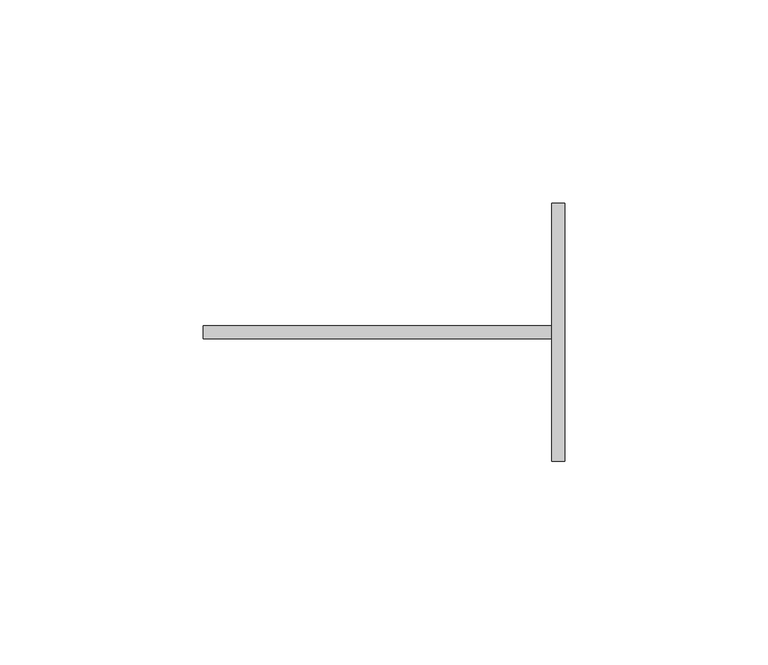
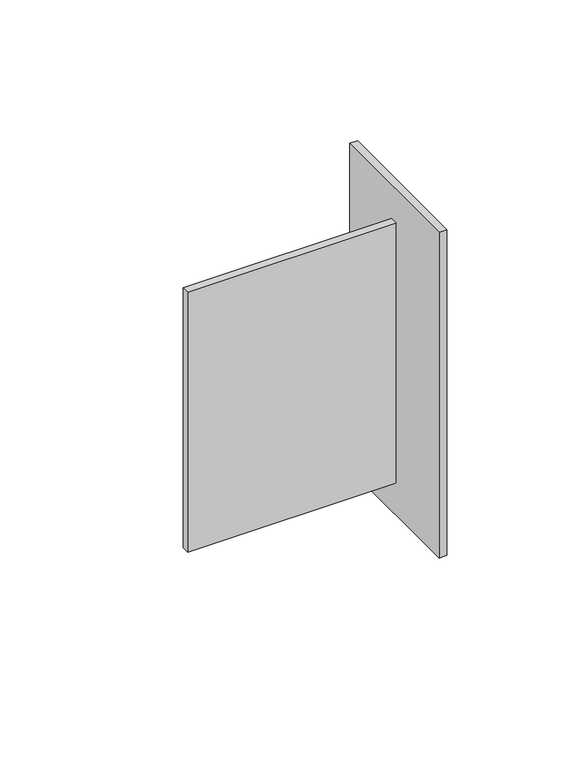
"""IFC4 building model written with IfcOpenShell, lengths in millimetres: proxy geometry, 060523 - W_P_C - Fastenings - Concealed Joist Ties:060523 - W_P_C - Fastenings - Concealed Joist Ties:154100 : 060523 - W_P_C - Fastenings - Concealed Joist Ties:060523 - W_P_C - Fastenings - Concealed Joist Ties:154100."""

from ifc_helpers import new_model, si_unit, frame, origin, place, context, project, spatial, polyline, outline, extrude, source, transform, mapped, element, save


def generic_models_267029ac(model_context):
    return source(origin(), model_context, "Body", "SweptSolid", [
        extrude(outline(polyline([(-6667.621787, -3916.4007855), (-6667.621787, -3852.9007855), (-6664.446787, -3852.9007855), (-6664.446787, -3916.4007855), (-6667.621787, -3916.4007855)])), frame((0.0, 0.0, 3169.0018876), z_axis=(0.0, 0.0, 1.0), x_axis=(1.0, 0.0, 0.0)), (0.0, 0.0, 1.0), 141.2875),
        extrude(outline(polyline([(-6753.346787, -3886.2382855), (-6753.346787, -3883.0632855), (-6667.621787, -3883.0632855), (-6667.621787, -3886.2382855), (-6753.346787, -3886.2382855)])), frame((0.0, 0.0, 3183.2893876), z_axis=(0.0, 0.0, 1.0), x_axis=(1.0, 0.0, 0.0)), (0.0, 0.0, 1.0), 112.7125),
    ])


if __name__ == "__main__":
    model = new_model("IFC4")
    model_context = context("Model", 3, world=origin())
    ifc_project = project(units=[si_unit("LENGTHUNIT", "METRE", prefix="MILLI")], contexts=[model_context])
    site = spatial("IfcSite", under=ifc_project)
    building = spatial("IfcBuilding", under=site)
    placement = place(None, origin())
    generic_models_shape = generic_models_267029ac(model_context)
    element("IfcBuildingElementProxy", 1, Name="060523 - W_P_C - Fastenings - Concealed Joist Ties:060523 - W_P_C - Fastenings - Concealed Joist Ties:154100 : 060523 - W_P_C - Fastenings - Concealed Joist Ties:060523 - W_P_C - Fastenings - Concealed Joist Ties:154100", ObjectType="060523 - W_P_C - Fastenings - Concealed Joist Ties:060523 - W_P_C - Fastenings - Concealed Joist Ties:154100 : 060523 - W_P_C - Fastenings - Concealed Joist Ties:060523 - W_P_C - Fastenings - Concealed Joist Ties:154100", at=placement, inside=building, context=model_context, shape_type="MappedRepresentation", body=[
        mapped(generic_models_shape, transform((0.0, 0.0, 0.0), x_axis=(1.0, 0.0, 0.0), y_axis=(0.0, 1.0, 0.0), z_axis=(0.0, 0.0, 1.0))),
    ])
    save(model, "model.ifc")

# Revit data of these elements
# Type "060523 - W_P_C - Fastenings - Concealed Joist Ties:060523 - W_P_C - Fastenings - Concealed Joist Ties:154100 : 060523 - W_P_C - Fastenings - Concealed Joist Ties:060523 - W_P_C - Fastenings - Concealed Joist Ties:154100"
#   NameOverride = "060523 - W_P_C - Fastenings - Concealed Joist Ties:060523 - W_P_C - Fastenings - Concealed Joist Ties:154100"
#   ObjectTypeOverride = "060523 - W_P_C - Fastenings - Concealed Joist Ties:060523 - W_P_C - Fastenings - Concealed Joist Ties"
#   Reference = "060523 - W_P_C - Fastenings - Concealed Joist Ties"
#   Category = "Generic Models"
#   Tag = "154100"
# Element 1 (IfcBuildingElementProxy, "060523 - W_P_C - Fastenings - Concealed Joist Ties:060523 - W_P_C - Fastenings - Concealed Joist Ties:154100 : 060523 - W_P_C - Fastenings - Concealed Joist Ties:060523 - W_P_C - Fastenings - Concealed Joist Ties:154100")
#   Materials on its faces: "_BEAM HANGER (SEE STRUCT. DWGS) 6017"
# Materials
#   "_BEAM HANGER (SEE STRUCT. DWGS) 6017": class "Unassigned", colour RGB 191 191 191, transparency 0
